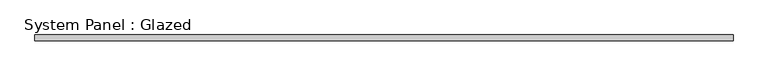
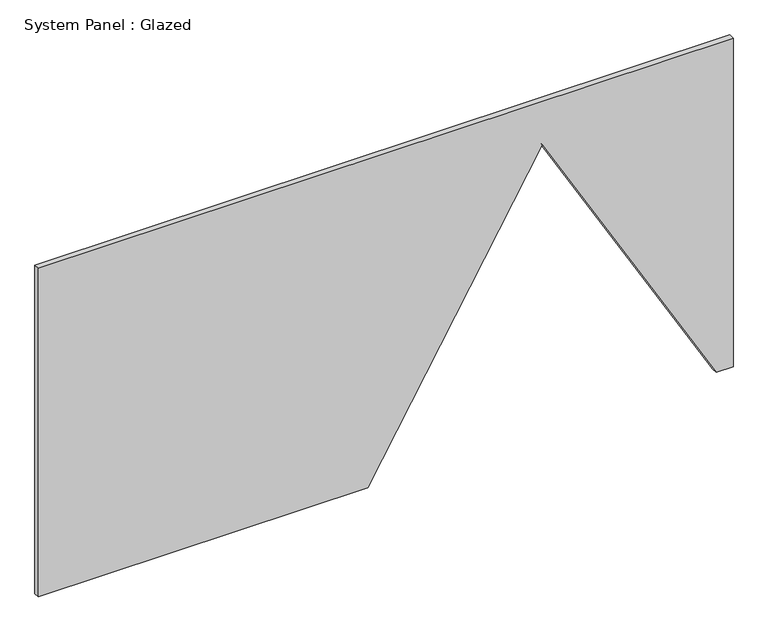
"""IFC4 building model written with IfcOpenShell, lengths in millimetres: plate geometry, System Panel : Glazed."""

from ifc_helpers import new_model, si_unit, frame, origin, place, context, project, spatial, polyline, outline, extrude, source, transform, mapped, element, save


def system_panel_glazed_8c6b7d14(model_context):
    return source(origin(), model_context, "Body", "SweptSolid", [
        extrude(outline(polyline([(0.0, -1500.0), (0.0, -76.4429578), (1301.5440949, 675.5392426), (0.0, 1426.4508999), (0.0, 1500.0), (1500.0, 1500.0), (1500.0, -1500.0), (0.0, -1500.0)])), frame((0.0, 24.5, 0.0), z_axis=(0.0, 1.0, 0.0), x_axis=(0.0, 0.0, 1.0)), (0.0, 0.0, 1.0), 25.0),
    ])


if __name__ == "__main__":
    model = new_model("IFC4")
    model_context = context("Model", 3, world=origin())
    ifc_project = project(units=[si_unit("LENGTHUNIT", "METRE", prefix="MILLI")], contexts=[model_context])
    site = spatial("IfcSite", under=ifc_project)
    building = spatial("IfcBuilding", under=site)
    placement = place(None, origin())
    system_panel_glazed_shape = system_panel_glazed_8c6b7d14(model_context)
    element("IfcPlate", 1, ObjectType="System Panel : Glazed", at=placement, inside=building, context=model_context, shape_type="MappedRepresentation", body=[
        mapped(system_panel_glazed_shape, transform((0.0, 0.0, 0.0), x_axis=(1.0, 0.0, 0.0), y_axis=(0.0, 1.0, 0.0), z_axis=(0.0, 0.0, 1.0))),
    ])
    save(model, "model.ifc")

# Revit data of these elements
# Project information
#   Project Issue Date = "Issue Date"
#   Project Status = "Project Status"
#   Client Name = "Owner"
#   Project Address = "Enter address here"
#   Project Name = "Project Name"
#   Project Number = "0001"
# Type "System Panel : Glazed"
#   Construction Type Id = "GSP4R"
#   Analytic Construction = "1/8 in Pilkington single glazing"
#   Visual Light Transmittance = 0.9
#   Solar Heat Gain Coefficient = 0.86
#   Heat Transfer Coefficient (U) = 6.7069 W/(m²·K)
#   Define Thermal Properties by = 1
# Element 1 (IfcPlate, "System Panel : Glazed")
#   Materials on its faces: "Glass"
# Materials
#   "Glass": class "Glass", colour RGB 0 128 192, transparency 0.9, Description = "Soda Lime Glass", Cost = 0
